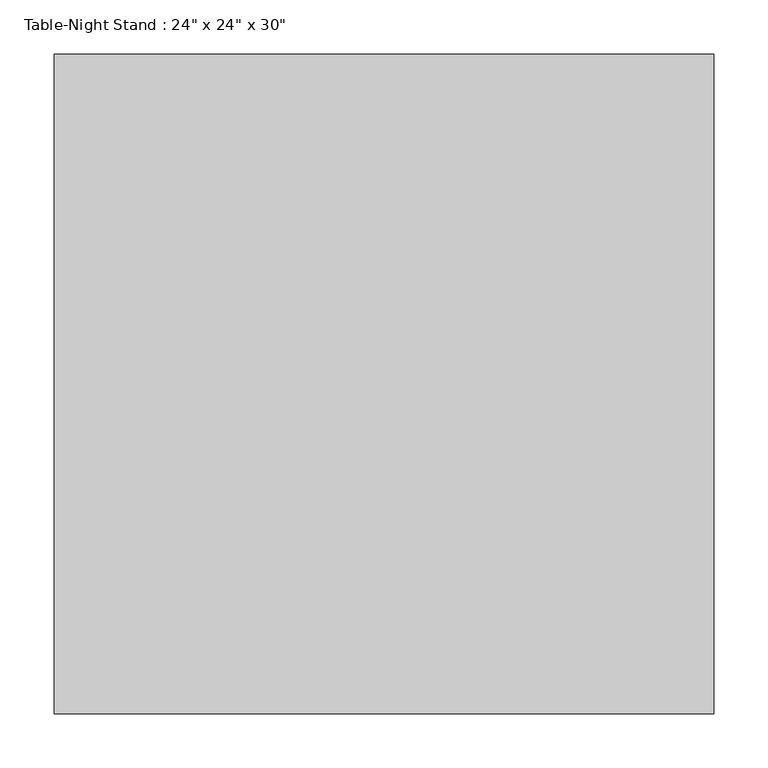
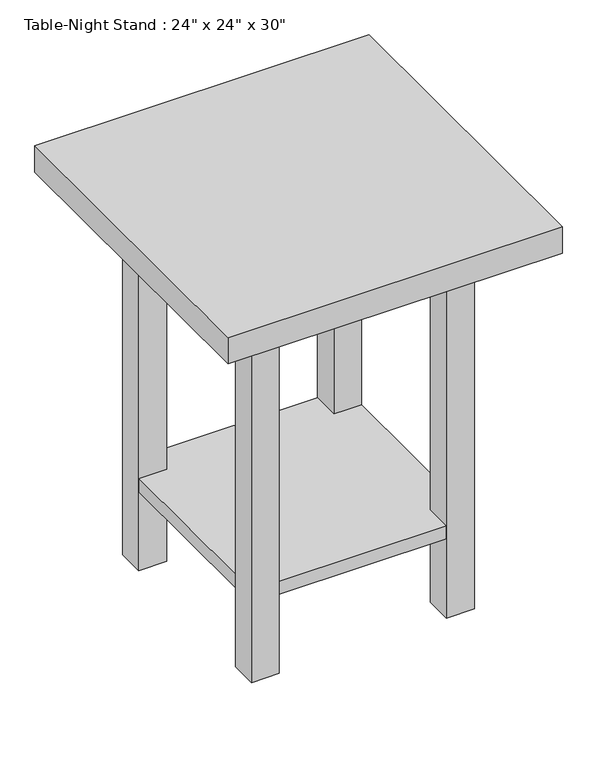
"""IFC4 building model written with IfcOpenShell, lengths in millimetres: furniture geometry."""

from ifc_helpers import new_model, si_unit, frame, origin, origin_with_axes, place, context, project, spatial, polyline, outline, extrude, source, transform, mapped, element, save


def furniture_910c7f7a(model_context):
    return source(origin(), model_context, "Body", "SweptSolid", [
        extrude(outline(polyline([(613.3336303, 0.0), (3.7336303, 0.0), (3.7336303, 609.6), (613.3336303, 609.6), (613.3336303, 0.0)])), frame((0.0, 0.0, 711.2), z_axis=(0.0, 0.0, 1.0), x_axis=(1.0, 0.0, 0.0)), (0.0, 0.0, 1.0), 50.8),
        extrude(outline(polyline([(156.1336303, 508.0), (156.1336303, 457.2), (105.3336303, 457.2), (105.3336303, 508.0), (156.1336303, 508.0)])), origin_with_axes(), (0.0, 0.0, 1.0), 711.2),
        extrude(outline(polyline([(156.1336303, 152.4), (156.1336303, 101.6), (105.3336303, 101.6), (105.3336303, 152.4), (156.1336303, 152.4)])), origin_with_axes(), (0.0, 0.0, 1.0), 711.2),
        extrude(outline(polyline([(511.7336303, 508.0), (511.7336303, 457.2), (460.9336303, 457.2), (460.9336303, 508.0), (511.7336303, 508.0)])), origin_with_axes(), (0.0, 0.0, 1.0), 711.2),
        extrude(outline(polyline([(511.7336303, 152.4), (511.7336303, 101.6), (460.9336303, 101.6), (460.9336303, 152.4), (511.7336303, 152.4)])), origin_with_axes(), (0.0, 0.0, 1.0), 711.2),
        extrude(outline(polyline([(156.1336303, 508.0), (460.9336303, 508.0), (460.9336303, 457.2), (511.7336303, 457.2), (511.7336303, 152.4), (460.9336303, 152.4), (460.9336303, 101.6), (156.1336303, 101.6), (156.1336303, 152.4), (105.3336303, 152.4), (105.3336303, 457.2), (156.1336303, 457.2), (156.1336303, 508.0)])), frame((0.0, 0.0, 152.4), z_axis=(0.0, 0.0, 1.0), x_axis=(1.0, 0.0, 0.0)), (0.0, 0.0, 1.0), 25.4),
    ])


if __name__ == "__main__":
    model = new_model("IFC4")
    model_context = context("Model", 3, world=origin())
    ifc_project = project(units=[si_unit("LENGTHUNIT", "METRE", prefix="MILLI")], contexts=[model_context])
    site = spatial("IfcSite", under=ifc_project)
    building = spatial("IfcBuilding", under=site)
    placement = place(None, origin())
    furniture_shape = furniture_910c7f7a(model_context)
    element("IfcFurniture", 1, ObjectType="Table-Night Stand : 24\" x 24\" x 30\"", at=placement, inside=building, context=model_context, shape_type="MappedRepresentation", body=[
        mapped(furniture_shape, transform((0.0, 0.0, 0.0), x_axis=(1.0, 0.0, 0.0), y_axis=(0.0, 1.0, 0.0), z_axis=(0.0, 0.0, 1.0))),
    ])
    save(model, "model.ifc")

# Revit data of these elements
# Type "Table-Night Stand : 24\" x 24\" x 30\""
#   Assembly Code = "E2020200"
#   Depth = 2' - 0"
#   Height = 2' - 6"
#   Width = 2' - 0"
#   Base Material = Birch
#   Top Material = Laminate, Ivory, Matte
#   Default Elevation = 0
# Element 1 (IfcFurniture, "Table-Night Stand : 24\" x 24\" x 30\"")
#   Materials on its faces: "Birch", "Laminate, Ivory, Matte"
# Materials
#   "Birch": class "Wood", colour RGB 224 178 126, transparency 0, Description = "Betula Alleghaniensis", Cost = 0
#   "Laminate, Ivory, Matte": class "Plastic", colour RGB 247 247 239, transparency 0, Description = "Plastic Laminate - Ivory, Matte", Cost = 0
